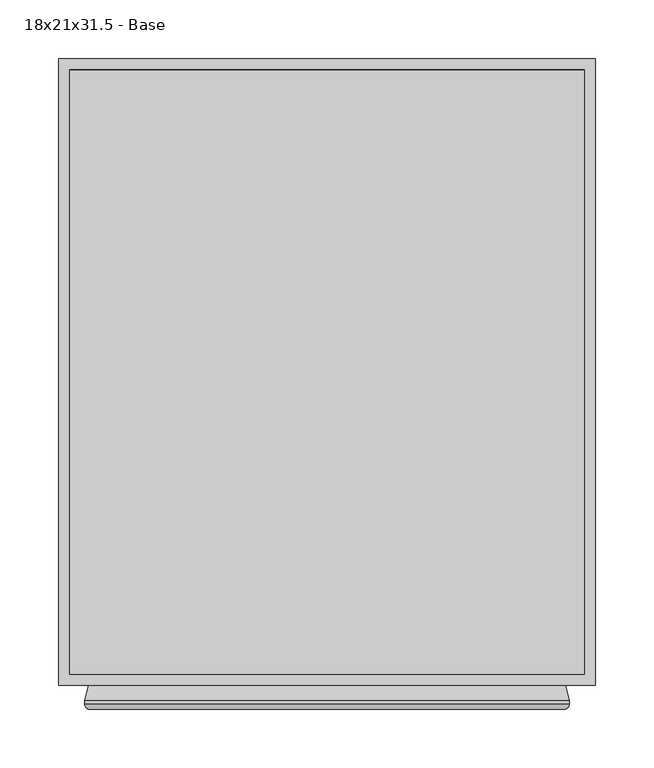
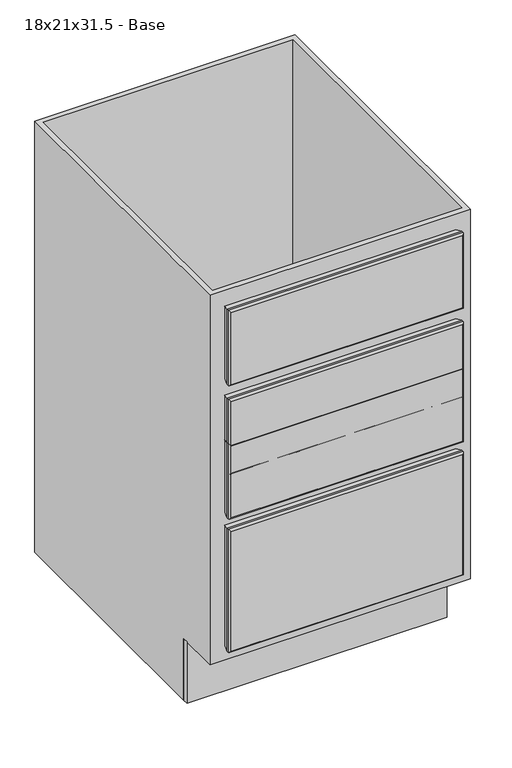
"""IFC4 building model written with IfcOpenShell, lengths in millimetres: furniture geometry, Cabinet-Base-Merillat-Four_Drawer-Marlin : 18x21x31.5 - Base."""

from ifc_helpers import new_model, si_unit, frame, origin, origin_with_axes, place, context, project, spatial, polyline, ellipse_curve, outline, extrude, faceted_brep, source, transform, mapped, element, save
from ifc_brep_helpers import plane_surface, cylinder_surface, advanced_brep


def furniture_18x21x31_5_base_3707efa4(model_context):
    return source(origin(), model_context, "Body", "SolidModel", [
        advanced_brep(
        [(-184.5408026, -629.92, 365.2035075), (-184.5408026, -629.92, 142.7964925), (222.0162124, -629.92, 142.7964925), (222.0162124, -629.92, 365.2035075), (-184.1320951, -609.6, 143.2052), (-184.1320951, -609.6, 364.7948), (221.6075049, -609.6, 364.7948), (221.6075049, -609.6, 143.2052), (-187.6372951, -625.4496, 368.3), (-187.6372951, -622.681, 368.3), (-187.6372951, -622.681, 139.7), (-187.6372951, -625.4496, 139.7), (225.1127049, -622.681, 139.7), (225.1127049, -625.4496, 139.7), (225.1127049, -622.681, 368.3), (225.1127049, -625.4496, 368.3)],
        [
            (0, 1),
            (1, 2),
            (2, 3),
            (3, 0),
            (4, 5),
            (5, 6),
            (6, 7),
            (7, 4),
            (8, 9),
            (9, 10),
            (10, 11),
            (11, 8),
            (10, 12),
            (12, 13),
            (13, 11),
            (12, 14),
            (14, 15),
            (15, 13),
            (8, 15),
            (14, 9),
            (11, 1, ellipse_curve(frame((-182.8620951, -625.4496, 144.4752), z_axis=(-0.7071067811865475, 0.0, 0.7071067811865475), x_axis=(-0.7071067811865474, 0.0, -0.7071067811865476)), 6.7531526, 4.7752)),
            (0, 8, ellipse_curve(frame((-182.8620951, -625.4496, 363.5248), z_axis=(-0.7071067811865475, 0.0, -0.7071067811865475), x_axis=(0.7071067811865474, 0.0, -0.7071067811865476)), 6.7531526, 4.7752)),
            (4, 10),
            (9, 5),
            (13, 2, ellipse_curve(frame((220.3375049, -625.4496, 144.4752), z_axis=(-0.7071067811865475, 0.0, -0.7071067811865475), x_axis=(0.7071067811865476, 0.0, -0.7071067811865474)), 6.7531526, 4.7752)),
            (7, 12),
            (15, 3, ellipse_curve(frame((220.3375049, -625.4496, 363.5248), z_axis=(0.7071067811865475, 0.0, -0.7071067811865475), x_axis=(0.7071067811865474, 0.0, 0.7071067811865476)), 6.7531526, 4.7752)),
            (6, 14),
        ],
        [
            plane_surface(frame((-187.6372951, -629.92, 368.3), z_axis=(0.0, -1.0, 0.0), x_axis=(0.0, 0.0, -1.0))),
            plane_surface(frame((-187.6372951, -609.6, 368.3), z_axis=(0.0, 1.0, 0.0), x_axis=(0.0, 0.0, 1.0))),
            plane_surface(frame((-187.6372951, -629.92, 368.3), z_axis=(-1.0, 0.0, 0.0), x_axis=(0.0, 1.0, 0.0))),
            plane_surface(frame((-187.6372951, -629.92, 139.7), z_axis=(0.0, 0.0, -1.0), x_axis=(0.0, 1.0, 0.0))),
            plane_surface(frame((225.1127049, -629.92, 139.7), z_axis=(1.0, 0.0, 0.0), x_axis=(0.0, 1.0, 0.0))),
            plane_surface(frame((225.1127049, -629.92, 368.3), z_axis=(0.0, 0.0, 1.0), x_axis=(0.0, 1.0, 0.0))),
            cylinder_surface(frame((-182.8620951, -625.4496, 368.3), z_axis=(0.0, 0.0, -1.0), x_axis=(0.0, 1.0, 0.0)), 4.7752),
            plane_surface(frame((-187.6372951, -622.681, 368.3), z_axis=(-0.9659229350723619, 0.25882983502910506, 0.0), x_axis=(0.0, 0.0, -1.0))),
            cylinder_surface(frame((-187.6372951, -625.4496, 144.4752), z_axis=(1.0, 0.0, 0.0), x_axis=(0.0, 1.0, 0.0)), 4.7752),
            plane_surface(frame((-187.6372951, -622.681, 139.7), z_axis=(0.0, 0.25882983502910506, -0.9659229350723619), x_axis=(1.0, 0.0, 0.0))),
            cylinder_surface(frame((220.3375049, -625.4496, 139.7), z_axis=(0.0, 0.0, 1.0), x_axis=(0.0, 1.0, 0.0)), 4.7752),
            plane_surface(frame((225.1127049, -622.681, 139.7), z_axis=(0.9659229350723619, 0.25882983502910506, 0.0), x_axis=(0.0, 0.0, 1.0))),
            cylinder_surface(frame((225.1127049, -625.4496, 363.5248), z_axis=(-1.0, 0.0, 0.0), x_axis=(0.0, 1.0, 0.0)), 4.7752),
            plane_surface(frame((225.1127049, -622.681, 368.3), z_axis=(0.0, 0.25882983502910506, 0.9659229350723619), x_axis=(-1.0, 0.0, 0.0))),
        ],
        [
            (0, [[1, 2, 3, 4]]),
            (1, [[5, 6, 7, 8]]),
            (2, [[9, 10, 11, 12]]),
            (3, [[-11, 13, 14, 15]]),
            (4, [[-14, 16, 17, 18]]),
            (5, [[-9, 19, -17, 20]]),
            (6, [[21, -1, 22, -12]]),
            (7, [[23, -10, 24, -5]]),
            (8, [[-21, -15, 25, -2]]),
            (9, [[-23, -8, 26, -13]]),
            (10, [[-25, -18, 27, -3]]),
            (11, [[-26, -7, 28, -16]]),
            (12, [[-22, -4, -27, -19]]),
            (13, [[-24, -20, -28, -6]]),
        ],
    ),
        advanced_brep(
        [(-184.5408026, -629.92, 523.9535075), (-184.5408026, -629.92, 390.4464925), (222.0162124, -629.92, 390.4464925), (222.0162124, -629.92, 523.9535075), (-184.1320951, -609.6, 390.8552), (-184.1320951, -609.6, 523.5448), (221.6075049, -609.6, 523.5448), (221.6075049, -609.6, 390.8552), (-187.6372951, -625.4496, 527.05), (-187.6372951, -622.681, 527.05), (-187.6372951, -622.681, 387.35), (-187.6372951, -625.4496, 387.35), (225.1127049, -622.681, 387.35), (225.1127049, -625.4496, 387.35), (225.1127049, -622.681, 527.05), (225.1127049, -625.4496, 527.05)],
        [
            (0, 1),
            (1, 2),
            (2, 3),
            (3, 0),
            (4, 5),
            (5, 6),
            (6, 7),
            (7, 4),
            (8, 9),
            (9, 10),
            (10, 11),
            (11, 8),
            (10, 12),
            (12, 13),
            (13, 11),
            (12, 14),
            (14, 15),
            (15, 13),
            (8, 15),
            (14, 9),
            (11, 1, ellipse_curve(frame((-182.8620951, -625.4496, 392.1252), z_axis=(-0.7071067811865475, 0.0, 0.7071067811865475), x_axis=(-0.7071067811865474, 0.0, -0.7071067811865476)), 6.7531526, 4.7752)),
            (0, 8, ellipse_curve(frame((-182.8620951, -625.4496, 522.2748), z_axis=(-0.7071067811865475, 0.0, -0.7071067811865475), x_axis=(0.7071067811865474, 0.0, -0.7071067811865476)), 6.7531526, 4.7752)),
            (4, 10),
            (9, 5),
            (13, 2, ellipse_curve(frame((220.3375049, -625.4496, 392.1252), z_axis=(-0.7071067811865475, 0.0, -0.7071067811865475), x_axis=(0.7071067811865476, 0.0, -0.7071067811865474)), 6.7531526, 4.7752)),
            (7, 12),
            (15, 3, ellipse_curve(frame((220.3375049, -625.4496, 522.2748), z_axis=(0.7071067811865475, 0.0, -0.7071067811865475), x_axis=(0.7071067811865474, 0.0, 0.7071067811865476)), 6.7531526, 4.7752)),
            (6, 14),
        ],
        [
            plane_surface(frame((-187.6372951, -629.92, 527.05), z_axis=(0.0, -1.0, 0.0), x_axis=(0.0, 0.0, -1.0))),
            plane_surface(frame((-187.6372951, -609.6, 527.05), z_axis=(0.0, 1.0, 0.0), x_axis=(0.0, 0.0, 1.0))),
            plane_surface(frame((-187.6372951, -629.92, 527.05), z_axis=(-1.0, 0.0, 0.0), x_axis=(0.0, 1.0, 0.0))),
            plane_surface(frame((-187.6372951, -629.92, 387.35), z_axis=(0.0, 0.0, -1.0), x_axis=(0.0, 1.0, 0.0))),
            plane_surface(frame((225.1127049, -629.92, 387.35), z_axis=(1.0, 0.0, 0.0), x_axis=(0.0, 1.0, 0.0))),
            plane_surface(frame((225.1127049, -629.92, 527.05), z_axis=(0.0, 0.0, 1.0), x_axis=(0.0, 1.0, 0.0))),
            cylinder_surface(frame((-182.8620951, -625.4496, 527.05), z_axis=(0.0, 0.0, -1.0), x_axis=(0.0, 1.0, 0.0)), 4.7752),
            plane_surface(frame((-187.6372951, -622.681, 527.05), z_axis=(-0.9659229350723619, 0.25882983502910506, 0.0), x_axis=(0.0, 0.0, -1.0))),
            cylinder_surface(frame((-187.6372951, -625.4496, 392.1252), z_axis=(1.0, 0.0, 0.0), x_axis=(0.0, 1.0, 0.0)), 4.7752),
            plane_surface(frame((-187.6372951, -622.681, 387.35), z_axis=(0.0, 0.25882983502910506, -0.9659229350723619), x_axis=(1.0, 0.0, 0.0))),
            cylinder_surface(frame((220.3375049, -625.4496, 387.35), z_axis=(0.0, 0.0, 1.0), x_axis=(0.0, 1.0, 0.0)), 4.7752),
            plane_surface(frame((225.1127049, -622.681, 387.35), z_axis=(0.9659229350723619, 0.25882983502910506, 0.0), x_axis=(0.0, 0.0, 1.0))),
            cylinder_surface(frame((225.1127049, -625.4496, 522.2748), z_axis=(-1.0, 0.0, 0.0), x_axis=(0.0, 1.0, 0.0)), 4.7752),
            plane_surface(frame((225.1127049, -622.681, 527.05), z_axis=(0.0, 0.25882983502910506, 0.9659229350723619), x_axis=(-1.0, 0.0, 0.0))),
        ],
        [
            (0, [[1, 2, 3, 4]]),
            (1, [[5, 6, 7, 8]]),
            (2, [[9, 10, 11, 12]]),
            (3, [[-11, 13, 14, 15]]),
            (4, [[-14, 16, 17, 18]]),
            (5, [[-9, 19, -17, 20]]),
            (6, [[21, -1, 22, -12]]),
            (7, [[23, -10, 24, -5]]),
            (8, [[-21, -15, 25, -2]]),
            (9, [[-23, -8, 26, -13]]),
            (10, [[-25, -18, 27, -3]]),
            (11, [[-26, -7, 28, -16]]),
            (12, [[-22, -4, -27, -19]]),
            (13, [[-24, -20, -28, -6]]),
        ],
    ),
        advanced_brep(
        [(-184.5408026, -629.92, 606.5035075), (-184.5408026, -629.92, 472.9964925), (222.0162124, -629.92, 472.9964925), (222.0162124, -629.92, 606.5035075), (-184.1320951, -609.6, 473.4052), (-184.1320951, -609.6, 606.0948), (221.6075049, -609.6, 606.0948), (221.6075049, -609.6, 473.4052), (-187.6372951, -625.4496, 609.6), (-187.6372951, -622.681, 609.6), (-187.6372951, -622.681, 469.9), (-187.6372951, -625.4496, 469.9), (225.1127049, -622.681, 469.9), (225.1127049, -625.4496, 469.9), (225.1127049, -622.681, 609.6), (225.1127049, -625.4496, 609.6)],
        [
            (0, 1),
            (1, 2),
            (2, 3),
            (3, 0),
            (4, 5),
            (5, 6),
            (6, 7),
            (7, 4),
            (8, 9),
            (9, 10),
            (10, 11),
            (11, 8),
            (10, 12),
            (12, 13),
            (13, 11),
            (12, 14),
            (14, 15),
            (15, 13),
            (8, 15),
            (14, 9),
            (11, 1, ellipse_curve(frame((-182.8620951, -625.4496, 474.6752), z_axis=(-0.7071067811865475, 0.0, 0.7071067811865475), x_axis=(-0.7071067811865474, 0.0, -0.7071067811865476)), 6.7531526, 4.7752)),
            (0, 8, ellipse_curve(frame((-182.8620951, -625.4496, 604.8248), z_axis=(-0.7071067811865475, 0.0, -0.7071067811865475), x_axis=(0.7071067811865474, 0.0, -0.7071067811865477)), 6.7531526, 4.7752)),
            (4, 10),
            (9, 5),
            (13, 2, ellipse_curve(frame((220.3375049, -625.4496, 474.6752), z_axis=(-0.7071067811865475, 0.0, -0.7071067811865475), x_axis=(0.7071067811865476, 0.0, -0.7071067811865474)), 6.7531526, 4.7752)),
            (7, 12),
            (15, 3, ellipse_curve(frame((220.3375049, -625.4496, 604.8248), z_axis=(0.7071067811865475, 0.0, -0.7071067811865475), x_axis=(0.7071067811865474, 0.0, 0.7071067811865476)), 6.7531526, 4.7752)),
            (6, 14),
        ],
        [
            plane_surface(frame((-187.6372951, -629.92, 609.6), z_axis=(0.0, -1.0, 0.0), x_axis=(0.0, 0.0, -1.0))),
            plane_surface(frame((-187.6372951, -609.6, 609.6), z_axis=(0.0, 1.0, 0.0), x_axis=(0.0, 0.0, 1.0))),
            plane_surface(frame((-187.6372951, -629.92, 609.6), z_axis=(-1.0, 0.0, 0.0), x_axis=(0.0, 1.0, 0.0))),
            plane_surface(frame((-187.6372951, -629.92, 469.9), z_axis=(0.0, 0.0, -1.0), x_axis=(0.0, 1.0, 0.0))),
            plane_surface(frame((225.1127049, -629.92, 469.9), z_axis=(1.0, 0.0, 0.0), x_axis=(0.0, 1.0, 0.0))),
            plane_surface(frame((225.1127049, -629.92, 609.6), z_axis=(0.0, 0.0, 1.0), x_axis=(0.0, 1.0, 0.0))),
            cylinder_surface(frame((-182.8620951, -625.4496, 609.6), z_axis=(0.0, 0.0, -1.0), x_axis=(0.0, 1.0, 0.0)), 4.7752),
            plane_surface(frame((-187.6372951, -622.681, 609.6), z_axis=(-0.9659229350723619, 0.25882983502910506, 0.0), x_axis=(0.0, 0.0, -1.0))),
            cylinder_surface(frame((-187.6372951, -625.4496, 474.6752), z_axis=(1.0, 0.0, 0.0), x_axis=(0.0, 1.0, 0.0)), 4.7752),
            plane_surface(frame((-187.6372951, -622.681, 469.9), z_axis=(0.0, 0.25882983502910506, -0.9659229350723619), x_axis=(1.0, 0.0, 0.0))),
            cylinder_surface(frame((220.3375049, -625.4496, 469.9), z_axis=(0.0, 0.0, 1.0), x_axis=(0.0, 1.0, 0.0)), 4.7752),
            plane_surface(frame((225.1127049, -622.681, 469.9), z_axis=(0.9659229350723619, 0.25882983502910506, 0.0), x_axis=(0.0, 0.0, 1.0))),
            cylinder_surface(frame((225.1127049, -625.4496, 604.8248), z_axis=(-1.0, 0.0, 0.0), x_axis=(0.0, 1.0, 0.0)), 4.7752),
            plane_surface(frame((225.1127049, -622.681, 609.6), z_axis=(0.0, 0.25882983502910506, 0.9659229350723619), x_axis=(-1.0, 0.0, 0.0))),
        ],
        [
            (0, [[1, 2, 3, 4]]),
            (1, [[5, 6, 7, 8]]),
            (2, [[9, 10, 11, 12]]),
            (3, [[-11, 13, 14, 15]]),
            (4, [[-14, 16, 17, 18]]),
            (5, [[-9, 19, -17, 20]]),
            (6, [[21, -1, 22, -12]]),
            (7, [[23, -10, 24, -5]]),
            (8, [[-21, -15, 25, -2]]),
            (9, [[-23, -8, 26, -13]]),
            (10, [[-25, -18, 27, -3]]),
            (11, [[-26, -7, 28, -16]]),
            (12, [[-22, -4, -27, -19]]),
            (13, [[-24, -20, -28, -6]]),
        ],
    ),
        advanced_brep(
        [(-184.5408026, -629.92, 771.6035075), (-184.5408026, -629.92, 638.0964925), (222.0162124, -629.92, 638.0964925), (222.0162124, -629.92, 771.6035075), (-184.1320951, -609.6, 638.5052), (-184.1320951, -609.6, 771.1948), (221.6075049, -609.6, 771.1948), (221.6075049, -609.6, 638.5052), (-187.6372951, -625.4496, 774.7), (-187.6372951, -622.681, 774.7), (-187.6372951, -622.681, 635.0), (-187.6372951, -625.4496, 635.0), (225.1127049, -622.681, 635.0), (225.1127049, -625.4496, 635.0), (225.1127049, -622.681, 774.7), (225.1127049, -625.4496, 774.7)],
        [
            (0, 1),
            (1, 2),
            (2, 3),
            (3, 0),
            (4, 5),
            (5, 6),
            (6, 7),
            (7, 4),
            (8, 9),
            (9, 10),
            (10, 11),
            (11, 8),
            (10, 12),
            (12, 13),
            (13, 11),
            (12, 14),
            (14, 15),
            (15, 13),
            (8, 15),
            (14, 9),
            (11, 1, ellipse_curve(frame((-182.8620951, -625.4496, 639.7752), z_axis=(-0.7071067811865475, 0.0, 0.7071067811865475), x_axis=(-0.7071067811865474, 0.0, -0.7071067811865476)), 6.7531526, 4.7752)),
            (0, 8, ellipse_curve(frame((-182.8620951, -625.4496, 769.9248), z_axis=(-0.7071067811865475, 0.0, -0.7071067811865475), x_axis=(0.7071067811865474, 0.0, -0.7071067811865477)), 6.7531526, 4.7752)),
            (4, 10),
            (9, 5),
            (13, 2, ellipse_curve(frame((220.3375049, -625.4496, 639.7752), z_axis=(-0.7071067811865475, 0.0, -0.7071067811865475), x_axis=(0.7071067811865476, 0.0, -0.7071067811865474)), 6.7531526, 4.7752)),
            (7, 12),
            (15, 3, ellipse_curve(frame((220.3375049, -625.4496, 769.9248), z_axis=(0.7071067811865475, 0.0, -0.7071067811865475), x_axis=(0.7071067811865474, 0.0, 0.7071067811865476)), 6.7531526, 4.7752)),
            (6, 14),
        ],
        [
            plane_surface(frame((-187.6372951, -629.92, 774.7), z_axis=(0.0, -1.0, 0.0), x_axis=(0.0, 0.0, -1.0))),
            plane_surface(frame((-187.6372951, -609.6, 774.7), z_axis=(0.0, 1.0, 0.0), x_axis=(0.0, 0.0, 1.0))),
            plane_surface(frame((-187.6372951, -629.92, 774.7), z_axis=(-1.0, 0.0, 0.0), x_axis=(0.0, 1.0, 0.0))),
            plane_surface(frame((-187.6372951, -629.92, 635.0), z_axis=(0.0, 0.0, -1.0), x_axis=(0.0, 1.0, 0.0))),
            plane_surface(frame((225.1127049, -629.92, 635.0), z_axis=(1.0, 0.0, 0.0), x_axis=(0.0, 1.0, 0.0))),
            plane_surface(frame((225.1127049, -629.92, 774.7), z_axis=(0.0, 0.0, 1.0), x_axis=(0.0, 1.0, 0.0))),
            cylinder_surface(frame((-182.8620951, -625.4496, 774.7), z_axis=(0.0, 0.0, -1.0), x_axis=(0.0, 1.0, 0.0)), 4.7752),
            plane_surface(frame((-187.6372951, -622.681, 774.7), z_axis=(-0.9659229350723619, 0.25882983502910506, 0.0), x_axis=(0.0, 0.0, -1.0))),
            cylinder_surface(frame((-187.6372951, -625.4496, 639.7752), z_axis=(1.0, 0.0, 0.0), x_axis=(0.0, 1.0, 0.0)), 4.7752),
            plane_surface(frame((-187.6372951, -622.681, 635.0), z_axis=(0.0, 0.25882983502910506, -0.9659229350723619), x_axis=(1.0, 0.0, 0.0))),
            cylinder_surface(frame((220.3375049, -625.4496, 635.0), z_axis=(0.0, 0.0, 1.0), x_axis=(0.0, 1.0, 0.0)), 4.7752),
            plane_surface(frame((225.1127049, -622.681, 635.0), z_axis=(0.9659229350723619, 0.25882983502910506, 0.0), x_axis=(0.0, 0.0, 1.0))),
            cylinder_surface(frame((225.1127049, -625.4496, 769.9248), z_axis=(-1.0, 0.0, 0.0), x_axis=(0.0, 1.0, 0.0)), 4.7752),
            plane_surface(frame((225.1127049, -622.681, 774.7), z_axis=(0.0, 0.25882983502910506, 0.9659229350723619), x_axis=(-1.0, 0.0, 0.0))),
        ],
        [
            (0, [[1, 2, 3, 4]]),
            (1, [[5, 6, 7, 8]]),
            (2, [[9, 10, 11, 12]]),
            (3, [[-11, 13, 14, 15]]),
            (4, [[-14, 16, 17, 18]]),
            (5, [[-9, 19, -17, 20]]),
            (6, [[21, -1, 22, -12]]),
            (7, [[23, -10, 24, -5]]),
            (8, [[-21, -15, 25, -2]]),
            (9, [[-23, -8, 26, -13]]),
            (10, [[-25, -18, 27, -3]]),
            (11, [[-26, -7, 28, -16]]),
            (12, [[-22, -4, -27, -19]]),
            (13, [[-24, -20, -28, -6]]),
        ],
    ),
        extrude(outline(polyline([(247.3377049, -529.43125), (247.3377049, -538.95625), (-209.8622951, -538.95625), (-209.8622951, -529.43125), (247.3377049, -529.43125)])), origin_with_axes(), (0.0, 0.0, 1.0), 114.3),
        faceted_brep([(247.3377049, -76.2, 0.0), (247.3377049, -529.43125, 0.0), (237.8127049, -529.43125, 0.0), (237.8127049, -85.725, 0.0), (-200.3372951, -85.725, 0.0), (-200.3372951, -529.43125, 0.0), (-209.8622951, -529.43125, 0.0), (-209.8622951, -76.2, 0.0), (-209.8622951, -76.2, 800.1), (247.3377049, -76.2, 800.1), (-209.8622951, -529.43125, 114.3), (-209.8622951, -609.6, 114.3), (-209.8622951, -609.6, 800.1), (247.3377049, -609.6, 800.1), (247.3377049, -609.6, 114.3), (247.3377049, -529.43125, 114.3), (237.8127049, -529.43125, 114.3), (237.8127049, -85.725, 114.3), (237.8127049, -600.075, 800.1), (237.8127049, -85.725, 800.1), (237.8127049, -85.725, 119.0625), (237.8127049, -600.075, 119.0625), (-200.3372951, -85.725, 114.3), (-200.3372951, -529.43125, 114.3), (-200.3372951, -85.725, 800.1), (-200.3372951, -600.075, 800.1), (-200.3372951, -600.075, 119.0625), (-200.3372951, -85.725, 119.0625)], [[[0, 1, 2, 3, 4, 5, 6, 7]], [[0, 7, 8, 9]], [[7, 6, 10, 11, 12, 8]], [[1, 0, 9, 13, 14, 15]], [[3, 2, 16, 17]], [[18, 19, 20, 21]], [[5, 4, 22, 23]], [[24, 25, 26, 27]], [[4, 3, 17, 22]], [[19, 24, 27, 20]], [[9, 8, 12, 13], [19, 18, 25, 24]], [[14, 11, 10, 23, 22, 17, 16, 15]], [[13, 12, 11, 14]], [[25, 18, 21, 26]], [[6, 5, 23, 10]], [[2, 1, 15, 16]], [[21, 20, 27, 26]]]),
    ])


if __name__ == "__main__":
    model = new_model("IFC4")
    model_context = context("Model", 3, world=origin())
    ifc_project = project(units=[si_unit("LENGTHUNIT", "METRE", prefix="MILLI")], contexts=[model_context])
    site = spatial("IfcSite", under=ifc_project)
    building = spatial("IfcBuilding", under=site)
    placement = place(None, origin())
    furniture_18x21x31_5_base_shape = furniture_18x21x31_5_base_3707efa4(model_context)
    element("IfcFurniture", 1, ObjectType="Cabinet-Base-Merillat-Four_Drawer-Marlin : 18x21x31.5 - Base", at=placement, inside=building, context=model_context, shape_type="MappedRepresentation", body=[
        mapped(furniture_18x21x31_5_base_shape, transform((0.0, 0.0, 0.0), x_axis=(1.0, 0.0, 0.0), y_axis=(0.0, 1.0, 0.0), z_axis=(0.0, 0.0, 1.0))),
    ])
    save(model, "model.ifc")

# Revit data of these elements
# Type "Cabinet-Base-Merillat-Four_Drawer-Marlin : 18x21x31.5 - Base"
#   URL = "http://www.merillat.com"
#   Toe Kick Note = "Toe Kick Covering is not included. To be purchased Separately."
#   Product Line = "Express"
#   Product Page URL = "http://www.merillat.com//our-products/rooms/kitchen/"
#   Product Group = "Base Cabinet"
#   Product Documentation Link = "http://merillatbusiness.com/customer-resources/product-line-resources/merillat-classic/"
#   Model = "BD18-4D"
#   Manufacturer = "Merillat"
#   Finish = "Wood"
#   Description = "Base Four Drawer Cabinet"
#   Construction Type = "Base Four Drawer"
#   Cabinet Construction Note = "3/4 extension sliders on all three drawers when SST or PST construction is chosen"
#   Assembly Code = "C1030410"
#   Top and Bottom Spacing = 0' - 1"
#   Toe Kick Height = 0' - 4 1/2"
#   Toe Kick Depth = 0' - 2 25/32"
#   Cabinet Shell = 0' - 0 3/8"
#   Middle Drawer Spacing = 0' - 0 3/4"
#   Depth = 1' - 9"
#   Height = 2' - 7 1/2"
#   Width = 1' - 6"
#   Deep Cabinet Drawer Height = 0' - 9"
#   Cabinet Drawer Width = 1' - 4 1/4"
#   Cabinet Drawer Height = 0' - 5 1/2"
#   COBie.Type = no
#   Partial Overlay = yes
#   Full Overlay = no
#   Toe Kick Material = Wood - Merillat - Raw Particle Board
#   Door Drawer Material = Wood - Merillat - Pecan(1)
#   Cabinet Drawer Style = element 826866
#   Cabinet Material = Wood - Merillat - Pecan(1)
# Element 1 (IfcFurniture, "Cabinet-Base-Merillat-Four_Drawer-Marlin : 18x21x31.5 - Base")
#   Materials on its faces: "Wood - Merillat - Pecan(1)", "Wood - Merillat - Raw Particle Board"
# Materials
#   "Wood - Merillat - Raw Particle Board": class "Plastic", colour RGB 80 80 80, transparency 0, Description = "Plastic Laminate - Navy", Cost = 0
#   "Wood - Merillat - Pecan(1)": class "Wood", colour RGB 108 67 43, transparency 0, Cost = 0
